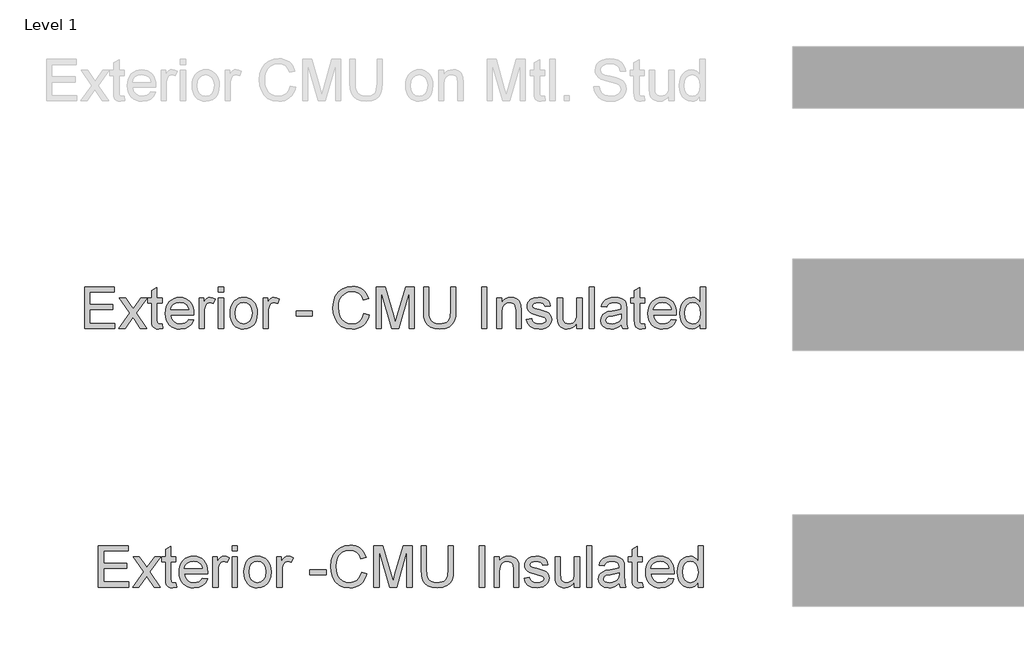
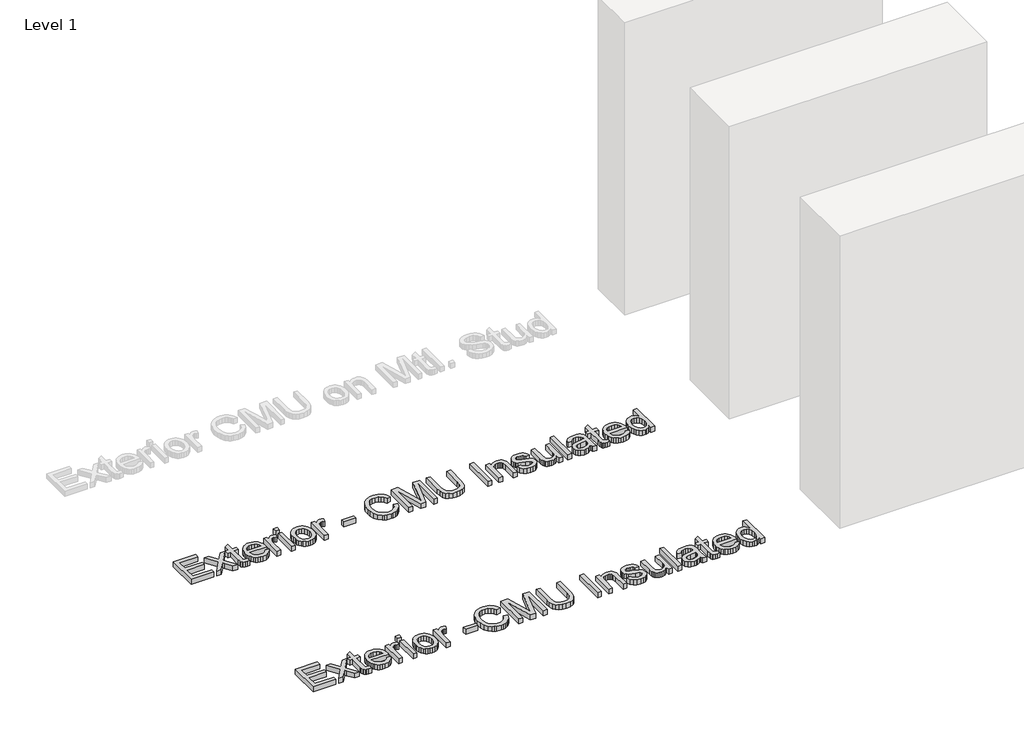
# One storey, part 20 of 42: 2 proxies.
"""IFC4 building model written with IfcOpenShell, lengths in millimetres."""

from ifc_helpers import new_model, si_unit, origin, origin_with_axes, place, context, project, spatial, polyline, outline, extrude, element, save

model = new_model("IFC4")

# Units and contexts
model_context = context("Model", 3, world=origin())
ifc_project = project(units=[si_unit("LENGTHUNIT", "METRE", prefix="MILLI")], contexts=[model_context])

# Site, building, storey
site = spatial("IfcSite", under=ifc_project)
building = spatial("IfcBuilding", under=site)
storey = spatial("IfcBuildingStorey", under=building, Name="Level 1", Elevation=0.0)

# Proxies
placement = place(None, origin())
element("IfcBuildingElementProxy", 1, Name="8\" Arial", ObjectType="8\" Arial", at=placement, inside=storey, context=model_context, shape_type="SweptSolid", body=[
    extrude(outline(polyline([(-4541.4204777, 3002.5650607), (-4541.4204777, 3307.1321548), (-4322.5128788, 3307.1321548), (-4322.5128788, 3269.061268), (-4503.3495909, 3269.061268), (-4503.3495909, 3178.642912), (-4332.0306005, 3178.642912), (-4332.0306005, 3140.5720252), (-4503.3495909, 3140.5720252), (-4503.3495909, 3040.6359475), (-4317.754018, 3040.6359475), (-4317.754018, 3002.5650607), (-4541.4204777, 3002.5650607)])), origin_with_axes(), (0.0, 0.0, 1.0), 50.8),
    extrude(outline(polyline([(-4289.2008529, 3002.5650607), (-4207.8540754, 3114.9931482), (-4284.4419921, 3226.2315204), (-4238.6379564, 3226.2315204), (-4201.6824277, 3172.6943359), (-4184.4315571, 3147.4128877), (-4169.4857598, 3168.0841895), (-4127.3995842, 3226.2315204), (-4081.5955486, 3226.2315204), (-4162.0500397, 3114.9931482), (-4084.5698366, 3002.5650607), (-4130.3738722, 3002.5650607), (-4176.9958371, 3070.1557562), (-4185.5469151, 3082.4990515), (-4243.3968173, 3002.5650607), (-4289.2008529, 3002.5650607)])), origin_with_axes(), (0.0, 0.0, 1.0), 50.8),
    extrude(outline(polyline([(-3970.3571763, 3034.3155854), (-3965.5983155, 3001.4497027), (-3994.0771233, 2997.8061999), (-4012.3504054, 2999.3862904), (-4025.9763624, 3004.126562), (-4035.6056199, 3011.4321569), (-4041.8888034, 3020.7082177), (-4045.3464132, 3036.639248), (-4046.4989498, 3063.9097513), (-4046.4989498, 3188.1606337), (-4075.0521149, 3188.1606337), (-4075.0521149, 3226.2315204), (-4046.4989498, 3226.2315204), (-4046.4989498, 3280.5866342), (-4008.4280631, 3302.9681516), (-4008.4280631, 3226.2315204), (-3970.3571763, 3226.2315204), (-3970.3571763, 3188.1606337), (-4008.4280631, 3188.1606337), (-4008.4280631, 3065.0251093), (-4006.4204187, 3045.3948083), (-3999.9141636, 3038.4424101), (-3986.9388321, 3035.8770867), (-3970.3571763, 3034.3155854)])), origin_with_axes(), (0.0, 0.0, 1.0), 50.8),
    extrude(outline(polyline([(-3775.6900249, 3069.1891126), (-3738.3627101, 3064.4302517), (-3751.8120688, 3036.3046406), (-3773.2734159, 3015.2801421), (-3802.2634295, 3002.1746854), (-3838.2987879, 2997.8061999), (-3861.9211411, 2999.6906902), (-3882.9688762, 3005.3441611), (-3901.4419932, 3014.7666126), (-3917.3404922, 3027.9580448), (-3930.1252834, 3044.5513188), (-3939.2572771, 3064.1792962), (-3944.7364734, 3086.8419767), (-3946.5628721, 3112.5393606), (-3944.7178841, 3139.1081179), (-3939.1829199, 3162.5259887), (-3929.9579797, 3182.7929733), (-3917.0430634, 3199.9090714), (-3901.1863904, 3213.5071445), (-3883.1361799, 3223.2200538), (-3862.892432, 3229.0477994), (-3840.4551467, 3230.9903813), (-3818.7405204, 3229.0524467), (-3799.1032485, 3223.2386431), (-3781.5433308, 3213.5489704), (-3766.0607674, 3199.9834286), (-3753.4223669, 3182.9045091), (-3744.394938, 3162.6747031), (-3738.9784807, 3139.2940109), (-3737.1729949, 3112.7624322), (-3737.3960665, 3102.5011385), (-3908.4919853, 3102.5011385), (-3901.9020784, 3074.0037413), (-3886.5937897, 3053.0536), (-3864.5004065, 3040.171215), (-3837.5552159, 3035.8770867), (-3817.2928787, 3037.8661418), (-3800.2279011, 3043.8333071), (-3786.3602832, 3054.1503687), (-3775.6900249, 3069.1891126)]), holes=[polyline([(-3908.4919853, 3140.5720252), (-3775.2438817, 3140.5720252), (-3780.3931178, 3160.685648), (-3790.4871078, 3175.0737664), (-3812.6827322, 3188.4580625), (-3840.6038611, 3192.9194945), (-3866.26639, 3189.3596435), (-3887.4860761, 3178.6800906), (-3902.2366858, 3162.0333723), (-3908.4919853, 3140.5720252)])]), origin_with_axes(), (0.0, 0.0, 1.0), 50.8),
    extrude(outline(polyline([(-3699.1021082, 3002.5650607), (-3699.1021082, 3226.2315204), (-3665.7900823, 3226.2315204), (-3665.7900823, 3193.1425661), (-3653.4839655, 3212.3267239), (-3642.1444924, 3223.6290184), (-3630.7678407, 3229.1500406), (-3618.3501882, 3230.9903813), (-3599.389102, 3228.0532719), (-3580.130587, 3219.2419436), (-3592.8456684, 3185.1119885), (-3606.2299645, 3190.967618), (-3619.6142606, 3192.9194945), (-3630.9816177, 3191.0419752), (-3641.1406702, 3185.4094173), (-3649.3478462, 3176.4493746), (-3654.8595737, 3164.5894011), (-3659.4883095, 3143.3232417), (-3661.0312214, 3120.123795), (-3661.0312214, 3002.5650607), (-3699.1021082, 3002.5650607)])), origin_with_axes(), (0.0, 0.0, 1.0), 50.8),
    extrude(outline(polyline([(-3556.3362828, 3269.061268), (-3556.3362828, 3307.1321548), (-3518.2653961, 3307.1321548), (-3518.2653961, 3269.061268), (-3556.3362828, 3269.061268)])), origin_with_axes(), (0.0, 0.0, 1.0), 50.8),
    extrude(outline(polyline([(-3556.3362828, 3002.5650607), (-3556.3362828, 3226.2315204), (-3518.2653961, 3226.2315204), (-3518.2653961, 3002.5650607), (-3556.3362828, 3002.5650607)])), origin_with_axes(), (0.0, 0.0, 1.0), 50.8),
    extrude(outline(polyline([(-3470.6767876, 3114.3982906), (-3468.6180226, 3143.3650676), (-3462.4417276, 3168.3258504), (-3452.1479027, 3189.280639), (-3437.7365477, 3206.2294335), (-3423.2275989, 3217.0623481), (-3407.2129168, 3224.8001443), (-3389.6925014, 3229.4428221), (-3370.6663527, 3230.9903813), (-3349.6627671, 3229.105891), (-3330.6714733, 3223.4524201), (-3313.6924713, 3214.0299685), (-3298.725761, 3200.8385364), (-3286.5102671, 3184.3242669), (-3277.7849143, 3164.9333031), (-3272.5497027, 3142.6656452), (-3270.8046321, 3117.521293), (-3273.890456, 3079.060031), (-3283.1479274, 3049.7818832), (-3298.3075017, 3027.8558036), (-3319.099634, 3011.4507462), (-3343.7955193, 3001.2173365), (-3370.6663527, 2997.8061999), (-3391.9766617, 2999.6837192), (-3411.1445538, 3005.3162772), (-3428.1700291, 3014.7038738), (-3443.0530876, 3027.846509), (-3455.1384563, 3044.5211112), (-3463.7708626, 3064.5046089), (-3468.9503064, 3087.797002), (-3470.6767876, 3114.3982906)]), holes=[polyline([(-3432.6059009, 3114.4726478), (-3428.2002367, 3080.0173799), (-3414.9832443, 3055.470209), (-3395.0926931, 3040.7753672), (-3370.6663527, 3035.8770867), (-3346.351548, 3040.8032512), (-3326.4981755, 3055.5817448), (-3313.281183, 3080.4542285), (-3308.8755189, 3115.662363), (-3313.309067, 3149.1138087), (-3326.6097113, 3173.3263721), (-3346.4909678, 3188.0212139), (-3370.6663527, 3192.9194945), (-3395.0926931, 3188.0398032), (-3414.9832443, 3173.4007293), (-3428.2002367, 3148.9093264), (-3432.6059009, 3114.4726478)])]), origin_with_axes(), (0.0, 0.0, 1.0), 50.8),
    extrude(outline(polyline([(-3227.9748845, 3002.5650607), (-3227.9748845, 3226.2315204), (-3194.6628586, 3226.2315204), (-3194.6628586, 3193.1425661), (-3182.3567419, 3212.3267239), (-3171.0172688, 3223.6290184), (-3159.6406171, 3229.1500406), (-3147.2229646, 3230.9903813), (-3128.2618784, 3228.0532719), (-3109.0033634, 3219.2419436), (-3121.7184447, 3185.1119885), (-3135.1027409, 3190.967618), (-3148.487037, 3192.9194945), (-3159.854394, 3191.0419752), (-3170.0134466, 3185.4094173), (-3178.2206226, 3176.4493746), (-3183.7323501, 3164.5894011), (-3188.3610859, 3143.3232417), (-3189.9039978, 3120.123795), (-3189.9039978, 3002.5650607), (-3227.9748845, 3002.5650607)])), origin_with_axes(), (0.0, 0.0, 1.0), 50.8),
    extrude(outline(polyline([(-2985.2729814, 3092.9834168), (-2985.2729814, 3131.0543035), (-2866.3014603, 3131.0543035), (-2866.3014603, 3092.9834168), (-2985.2729814, 3092.9834168)])), origin_with_axes(), (0.0, 0.0, 1.0), 50.8),
    extrude(outline(polyline([(-2485.5925927, 3110.829145), (-2447.521706, 3101.0139945), (-2455.0550199, 3077.338197), (-2465.0885946, 3056.6506296), (-2477.6224303, 3038.9512922), (-2492.6565268, 3024.2401847), (-2509.8516295, 3012.6753164), (-2528.8684835, 3004.4146961), (-2549.707089, 2999.4583239), (-2572.367446, 2997.8061999), (-2616.5263285, 3002.8067216), (-2635.1969569, 3009.0573738), (-2651.5950433, 3017.8082869), (-2678.4751714, 3042.2903952), (-2698.0682937, 3075.7325462), (-2710.0305084, 3115.0489161), (-2714.0179133, 3157.153681), (-2709.510008, 3201.5635191), (-2695.9862921, 3239.9132454), (-2674.1531591, 3270.9852606), (-2644.7170022, 3293.5619657), (-2609.8062965, 3307.3087532), (-2571.5495167, 3311.8910157), (-2549.7744753, 3310.408519), (-2529.8072432, 3305.9610289), (-2511.6478206, 3298.5485455), (-2495.2962074, 3288.1710686), (-2481.0219486, 3275.1027906), (-2469.0945888, 3259.6179036), (-2452.2805668, 3221.3983024), (-2490.3514536, 3212.3267239), (-2503.5498567, 3240.0898437), (-2521.5814779, 3259.1345818), (-2544.6693887, 3270.1487421), (-2573.0366608, 3273.8201289), (-2605.7352398, 3269.7490722), (-2632.5967785, 3257.5359019), (-2652.9799462, 3238.46328), (-2666.2434118, 3213.8138679), (-2673.5211229, 3185.948507), (-2675.9470265, 3157.2280382), (-2673.0749797, 3122.0570823), (-2664.458839, 3091.6449872), (-2649.7732919, 3067.1535842), (-2628.6930255, 3049.7447046), (-2603.4208719, 3039.3439911), (-2576.1596632, 3035.8770867), (-2544.3812545, 3040.5987689), (-2517.9007964, 3054.7638156), (-2497.9080041, 3078.2235125), (-2485.5925927, 3110.829145)])), origin_with_axes(), (0.0, 0.0, 1.0), 50.8),
    extrude(outline(polyline([(-2395.1742367, 3002.5650607), (-2395.1742367, 3307.1321548), (-2329.6655429, 3307.1321548), (-2267.3542087, 3092.4629164), (-2254.7878418, 3047.6255244), (-2241.180474, 3096.1807764), (-2179.9101407, 3307.1321548), (-2114.4014468, 3307.1321548), (-2114.4014468, 3002.5650607), (-2152.4723336, 3002.5650607), (-2152.4723336, 3269.061268), (-2228.9858931, 3002.5650607), (-2280.5897904, 3002.5650607), (-2357.1033499, 3269.061268), (-2357.1033499, 3002.5650607), (-2395.1742367, 3002.5650607)])), origin_with_axes(), (0.0, 0.0, 1.0), 50.8),
    extrude(outline(polyline([(-1847.9052395, 3307.1321548), (-1809.8343528, 3307.1321548), (-1809.8343528, 3131.4260896), (-1812.4182655, 3090.2786736), (-1820.1700037, 3058.5932115), (-1834.6510685, 3034.1482817), (-1857.4229612, 3014.7224631), (-1888.5414497, 3002.0352657), (-1928.0623019, 2997.8061999), (-1966.7187516, 3001.4868813), (-1997.6234631, 3012.5289256), (-2020.7857312, 3030.5512522), (-2036.2148503, 3055.1727802), (-2044.8867588, 3088.196672), (-2047.777395, 3131.4260896), (-2047.777395, 3307.1321548), (-2009.7065083, 3307.1321548), (-2009.7065083, 3132.7645192), (-2007.8289889, 3098.5509122), (-2002.196431, 3074.728724), (-1991.9909052, 3058.2307201), (-1976.3944823, 3045.9896659), (-1956.0577879, 3038.4052315), (-1931.6314475, 3035.8770867), (-1892.9099353, 3040.8776084), (-1878.4149284, 3047.1282606), (-1867.1637545, 3055.8791736), (-1858.7381542, 3068.1852904), (-1852.7198683, 3085.1015535), (-1847.9052395, 3132.7645192), (-1847.9052395, 3307.1321548)])), origin_with_axes(), (0.0, 0.0, 1.0), 50.8),
    extrude(outline(polyline([(-1619.479919, 3002.5650607), (-1619.479919, 3307.1321548), (-1581.4090322, 3307.1321548), (-1581.4090322, 3002.5650607), (-1619.479919, 3002.5650607)])), origin_with_axes(), (0.0, 0.0, 1.0), 50.8),
    extrude(outline(polyline([(-1510.0261195, 3002.5650607), (-1510.0261195, 3226.2315204), (-1471.9552328, 3226.2315204), (-1471.9552328, 3195.0014962), (-1458.7289457, 3210.7466334), (-1442.8443887, 3221.99316), (-1424.3015618, 3228.741076), (-1403.1004649, 3230.9903813), (-1384.3345664, 3229.1779245), (-1367.1487584, 3223.7405542), (-1352.816408, 3215.3567798), (-1342.6108822, 3204.7051108), (-1331.1970519, 3176.7096248), (-1329.1894074, 3139.9028104), (-1329.1894074, 3002.5650607), (-1367.2602942, 3002.5650607), (-1367.2602942, 3134.7721636), (-1371.647369, 3168.4559755), (-1377.7167756, 3178.4849029), (-1387.1508454, 3186.2645251), (-1399.2431852, 3191.2557522), (-1413.2874014, 3192.9194945), (-1435.585267, 3189.1830452), (-1454.5928264, 3177.9736972), (-1462.1888792, 3168.8231142), (-1467.6146312, 3156.3171625), (-1471.9552328, 3121.2391531), (-1471.9552328, 3002.5650607), (-1510.0261195, 3002.5650607)])), origin_with_axes(), (0.0, 0.0, 1.0), 50.8),
    extrude(outline(polyline([(-1291.1185207, 3069.1891126), (-1253.0476339, 3073.9479734), (-1247.04329, 3057.6637465), (-1235.4249774, 3045.6922371), (-1218.1183389, 3038.3308743), (-1195.0490174, 3035.8770867), (-1172.2585354, 3038.126392), (-1156.2345586, 3044.8743079), (-1146.7540155, 3054.6522798), (-1143.5938345, 3065.9917529), (-1146.7726048, 3075.6953676), (-1156.3089158, 3083.0939091), (-1195.4951606, 3093.9500604), (-1252.8245623, 3112.5765392), (-1267.3335111, 3121.9362518), (-1277.8457604, 3134.3260204), (-1284.231185, 3148.9557996), (-1286.3596598, 3165.0355443), (-1284.6494442, 3179.786154), (-1279.5187974, 3193.4028163), (-1271.4324518, 3205.3464417), (-1260.85514, 3215.0779403), (-1236.6518712, 3226.3430562), (-1203.8975243, 3230.9903813), (-1179.1179871, 3229.1221566), (-1157.5729882, 3223.5174826), (-1140.2477605, 3214.7247436), (-1128.1275368, 3203.292324), (-1120.0969591, 3188.3744106), (-1115.0406694, 3169.1251903), (-1153.1115562, 3164.3663295), (-1157.9168903, 3176.3471334), (-1167.4253173, 3185.3722387), (-1181.7297838, 3191.0326806), (-1200.9232362, 3192.9194945), (-1222.7842532, 3191.1163324), (-1237.3582646, 3185.7068461), (-1245.556146, 3177.89934), (-1248.2887731, 3168.9021187), (-1243.7529838, 3157.8228958), (-1229.5507585, 3149.4205321), (-1196.759233, 3141.3155972), (-1140.8797967, 3123.3955119), (-1126.1198923, 3114.8258445), (-1114.9291336, 3103.0959961), (-1107.8744942, 3088.168788), (-1105.5229477, 3070.0070418), (-1108.2834588, 3051.2318486), (-1116.564992, 3033.5720134), (-1130.0515293, 3018.4124391), (-1148.4270525, 3007.1380286), (-1170.622677, 3000.1391571), (-1195.5695178, 2997.8061999), (-1233.9564226, 3002.3048105), (-1261.970498, 3015.8006425), (-1280.671334, 3038.1449813), (-1291.1185207, 3069.1891126)])), origin_with_axes(), (0.0, 0.0, 1.0), 50.8),
    extrude(outline(polyline([(-919.9273748, 3002.5650607), (-919.9273748, 3041.0077335), (-933.7020462, 3022.1070625), (-949.7446123, 3008.6065833), (-968.0550729, 3000.5062957), (-988.6334282, 2997.8061999), (-1007.1762552, 2999.7023085), (-1024.4364204, 3005.3906344), (-1038.9174852, 3013.9417124), (-1049.123011, 3024.4260777), (-1055.9917574, 3037.1597484), (-1060.4624841, 3052.4587424), (-1062.6932001, 3087.8527699), (-1062.6932001, 3226.2315204), (-1024.6223134, 3226.2315204), (-1024.6223134, 3105.7728553), (-1022.3172402, 3066.9583965), (-1016.7683341, 3054.010949), (-1007.259907, 3044.1679145), (-994.4239952, 3037.9497936), (-978.8926349, 3035.8770867), (-962.4689882, 3037.9962669), (-947.1049316, 3044.3538075), (-934.4363236, 3054.3641457), (-926.0990224, 3067.4417184), (-921.4702867, 3085.3525091), (-919.9273748, 3109.8625013), (-919.9273748, 3226.2315204), (-881.856488, 3226.2315204), (-881.856488, 3002.5650607), (-919.9273748, 3002.5650607)])), origin_with_axes(), (0.0, 0.0, 1.0), 50.8),
    extrude(outline(polyline([(-829.5090187, 3002.5650607), (-829.5090187, 3307.1321548), (-791.438132, 3307.1321548), (-791.438132, 3002.5650607), (-829.5090187, 3002.5650607)])), origin_with_axes(), (0.0, 0.0, 1.0), 50.8),
    extrude(outline(polyline([(-591.5659765, 3031.1182258), (-609.7556067, 3015.521803), (-628.4843266, 3005.3162772), (-648.1796902, 2999.6837192), (-669.2692512, 2997.8061999), (-701.0848385, 3002.3233998), (-724.55383, 3015.8749997), (-739.0256001, 3036.453355), (-743.8495235, 3062.0508213), (-742.0277721, 3077.8331371), (-736.5625179, 3092.1654876), (-728.1322702, 3104.4344257), (-717.4155387, 3114.0265046), (-690.7584822, 3126.5185143), (-657.8182423, 3132.2440188), (-618.8922478, 3138.266952), (-591.7890481, 3145.3308861), (-591.5659765, 3153.807607), (-594.1870678, 3170.7982273), (-602.0503418, 3181.9146288), (-619.6358198, 3190.1682781), (-644.1365174, 3192.9194945), (-666.8154636, 3191.0884485), (-682.6535474, 3185.5953103), (-693.4539308, 3175.4362577), (-701.0197759, 3159.6074686), (-739.0906627, 3164.3663295), (-732.4821665, 3185.1863457), (-722.6205427, 3201.5449298), (-708.5856211, 3214.0555288), (-689.4572312, 3223.3315896), (-666.062597, 3229.0756834), (-639.2289421, 3230.9903813), (-613.4920561, 3229.298755), (-593.0902991, 3224.223876), (-577.7076532, 3216.5929683), (-567.0281003, 3207.2332557), (-559.9455769, 3195.6614163), (-555.3540198, 3181.3941284), (-553.4950897, 3148.0821025), (-553.4950897, 3100.7165657), (-551.5618025, 3034.5758356), (-543.9773681, 3002.5650607), (-582.0482548, 3002.5650607), (-588.1455453, 3015.8006425), (-591.5659765, 3031.1182258)]), holes=[polyline([(-591.5659765, 3107.2599993), (-652.9850243, 3095.5859188), (-685.7393712, 3089.4142712), (-700.5736327, 3079.3760491), (-705.7786368, 3064.7276805), (-702.9437685, 3053.4067967), (-694.4391637, 3044.1307359), (-680.4507153, 3037.940499), (-661.1643164, 3035.8770867), (-640.7160862, 3038.1542759), (-622.6472864, 3044.9858437), (-607.9989179, 3055.0519498), (-597.8119814, 3067.0327537), (-593.2947814, 3079.3760491), (-591.7890481, 3096.4782052), (-591.5659765, 3107.2599993)])]), origin_with_axes(), (0.0, 0.0, 1.0), 50.8),
    extrude(outline(polyline([(-420.2469861, 3034.3155854), (-415.4881252, 3001.4497027), (-443.9669331, 2997.8061999), (-462.2402152, 2999.3862904), (-475.8661722, 3004.126562), (-485.4954297, 3011.4321569), (-491.7786132, 3020.7082177), (-495.236223, 3036.639248), (-496.3887596, 3063.9097513), (-496.3887596, 3188.1606337), (-524.9419247, 3188.1606337), (-524.9419247, 3226.2315204), (-496.3887596, 3226.2315204), (-496.3887596, 3280.5866342), (-458.3178728, 3302.9681516), (-458.3178728, 3226.2315204), (-420.2469861, 3226.2315204), (-420.2469861, 3188.1606337), (-458.3178728, 3188.1606337), (-458.3178728, 3065.0251093), (-456.3102284, 3045.3948083), (-449.8039734, 3038.4424101), (-436.8286418, 3035.8770867), (-420.2469861, 3034.3155854)])), origin_with_axes(), (0.0, 0.0, 1.0), 50.8),
    extrude(outline(polyline([(-225.5798347, 3069.1891126), (-188.2525199, 3064.4302517), (-201.7018786, 3036.3046406), (-223.1632256, 3015.2801421), (-252.1532393, 3002.1746854), (-288.1885976, 2997.8061999), (-311.8109508, 2999.6906902), (-332.858686, 3005.3441611), (-351.331803, 3014.7666126), (-367.230302, 3027.9580448), (-380.0150932, 3044.5513188), (-389.1470869, 3064.1792962), (-394.6262831, 3086.8419767), (-396.4526819, 3112.5393606), (-394.6076938, 3139.1081179), (-389.0727297, 3162.5259887), (-379.8477895, 3182.7929733), (-366.9328732, 3199.9090714), (-351.0762001, 3213.5071445), (-333.0259897, 3223.2200538), (-312.7822418, 3229.0477994), (-290.3449565, 3230.9903813), (-268.6303302, 3229.0524467), (-248.9930582, 3223.2386431), (-231.4331405, 3213.5489704), (-215.9505772, 3199.9834286), (-203.3121767, 3182.9045091), (-194.2847478, 3162.6747031), (-188.8682905, 3139.2940109), (-187.0628047, 3112.7624322), (-187.2858763, 3102.5011385), (-358.3817951, 3102.5011385), (-351.7918882, 3074.0037413), (-336.4835995, 3053.0536), (-314.3902162, 3040.171215), (-287.4450256, 3035.8770867), (-267.1826884, 3037.8661418), (-250.1177109, 3043.8333071), (-236.250093, 3054.1503687), (-225.5798347, 3069.1891126)]), holes=[polyline([(-358.3817951, 3140.5720252), (-225.1336914, 3140.5720252), (-230.2829276, 3160.685648), (-240.3769176, 3175.0737664), (-262.572542, 3188.4580625), (-290.4936709, 3192.9194945), (-316.1561998, 3189.3596435), (-337.3758859, 3178.6800906), (-352.1264956, 3162.0333723), (-358.3817951, 3140.5720252)])]), origin_with_axes(), (0.0, 0.0, 1.0), 50.8),
    extrude(outline(polyline([(-10.9849534, 3002.5650607), (-10.9849534, 3038.4795887), (-22.3755471, 3020.6849811), (-36.1734552, 3007.9745471), (-52.3786776, 3000.3482867), (-70.9912144, 2997.8061999), (-95.6034478, 3001.4868813), (-118.1336796, 3012.5289256), (-137.2063016, 3030.1608768), (-151.4457056, 3053.611279), (-160.3128017, 3081.9320778), (-163.2685005, 3114.175219), (-160.545168, 3146.0186902), (-152.3751706, 3174.7763376), (-138.7678028, 3198.8123027), (-119.7323595, 3216.4907272), (-96.7095112, 3227.3654678), (-71.1399288, 3230.9903813), (-52.51345, 3228.3971739), (-36.0433301, 3220.6175518), (-22.0827656, 3208.6925157), (-10.9849534, 3193.6630665), (-10.9849534, 3307.1321548), (27.0859333, 3307.1321548), (27.0859333, 3002.5650607), (-10.9849534, 3002.5650607)]), holes=[polyline([(-125.1976137, 3114.3239334), (-120.9034854, 3079.8872548), (-108.0211003, 3055.3958518), (-89.3016751, 3040.7567779), (-67.496426, 3035.8770867), (-45.7004715, 3040.5337063), (-27.4550734, 3054.5035654), (-15.1024834, 3078.0469141), (-10.9849534, 3111.4240026), (-15.1768406, 3147.9147988), (-27.7525022, 3173.2148363), (-46.4626328, 3187.99333), (-69.0579272, 3192.9194945), (-91.0862479, 3188.1885176), (-109.1364584, 3173.995587), (-121.1823249, 3149.6157198), (-125.1976137, 3114.3239334)])]), origin_with_axes(), (0.0, 0.0, 1.0), 50.8),
])
element("IfcBuildingElementProxy", 2, Name="8\" Arial", ObjectType="8\" Arial", at=placement, inside=storey, context=model_context, shape_type="SweptSolid", body=[
    extrude(outline(polyline([(-4439.8204777, 1097.5650607), (-4439.8204777, 1402.1321548), (-4220.9128788, 1402.1321548), (-4220.9128788, 1364.061268), (-4401.7495909, 1364.061268), (-4401.7495909, 1273.642912), (-4230.4306005, 1273.642912), (-4230.4306005, 1235.5720252), (-4401.7495909, 1235.5720252), (-4401.7495909, 1135.6359475), (-4216.154018, 1135.6359475), (-4216.154018, 1097.5650607), (-4439.8204777, 1097.5650607)])), origin_with_axes(), (0.0, 0.0, 1.0), 50.8),
    extrude(outline(polyline([(-4187.6008529, 1097.5650607), (-4106.2540754, 1209.9931482), (-4182.8419921, 1321.2315204), (-4137.0379564, 1321.2315204), (-4100.0824277, 1267.6943359), (-4082.8315571, 1242.4128877), (-4067.8857598, 1263.0841895), (-4025.7995842, 1321.2315204), (-3979.9955486, 1321.2315204), (-4060.4500397, 1209.9931482), (-3982.9698366, 1097.5650607), (-4028.7738722, 1097.5650607), (-4075.3958371, 1165.1557562), (-4083.9469151, 1177.4990515), (-4141.7968173, 1097.5650607), (-4187.6008529, 1097.5650607)])), origin_with_axes(), (0.0, 0.0, 1.0), 50.8),
    extrude(outline(polyline([(-3868.7571763, 1129.3155854), (-3863.9983155, 1096.4497027), (-3892.4771233, 1092.8061999), (-3910.7504054, 1094.3862904), (-3924.3763624, 1099.126562), (-3934.0056199, 1106.4321569), (-3940.2888034, 1115.7082177), (-3943.7464132, 1131.639248), (-3944.8989498, 1158.9097513), (-3944.8989498, 1283.1606337), (-3973.4521149, 1283.1606337), (-3973.4521149, 1321.2315204), (-3944.8989498, 1321.2315204), (-3944.8989498, 1375.5866342), (-3906.8280631, 1397.9681516), (-3906.8280631, 1321.2315204), (-3868.7571763, 1321.2315204), (-3868.7571763, 1283.1606337), (-3906.8280631, 1283.1606337), (-3906.8280631, 1160.0251093), (-3904.8204187, 1140.3948083), (-3898.3141636, 1133.4424101), (-3885.3388321, 1130.8770867), (-3868.7571763, 1129.3155854)])), origin_with_axes(), (0.0, 0.0, 1.0), 50.8),
    extrude(outline(polyline([(-3674.0900249, 1164.1891126), (-3636.7627101, 1159.4302517), (-3650.2120688, 1131.3046406), (-3671.6734159, 1110.2801421), (-3700.6634295, 1097.1746854), (-3736.6987879, 1092.8061999), (-3760.3211411, 1094.6906902), (-3781.3688762, 1100.3441611), (-3799.8419932, 1109.7666126), (-3815.7404922, 1122.9580448), (-3828.5252834, 1139.5513188), (-3837.6572771, 1159.1792962), (-3843.1364734, 1181.8419767), (-3844.9628721, 1207.5393606), (-3843.1178841, 1234.1081179), (-3837.5829199, 1257.5259887), (-3828.3579797, 1277.7929733), (-3815.4430634, 1294.9090714), (-3799.5863904, 1308.5071445), (-3781.5361799, 1318.2200538), (-3761.292432, 1324.0477994), (-3738.8551467, 1325.9903813), (-3717.1405204, 1324.0524467), (-3697.5032485, 1318.2386431), (-3679.9433308, 1308.5489704), (-3664.4607674, 1294.9834286), (-3651.8223669, 1277.9045091), (-3642.794938, 1257.6747031), (-3637.3784807, 1234.2940109), (-3635.5729949, 1207.7624322), (-3635.7960665, 1197.5011385), (-3806.8919853, 1197.5011385), (-3800.3020784, 1169.0037413), (-3784.9937897, 1148.0536), (-3762.9004065, 1135.171215), (-3735.9552159, 1130.8770867), (-3715.6928787, 1132.8661418), (-3698.6279011, 1138.8333071), (-3684.7602832, 1149.1503687), (-3674.0900249, 1164.1891126)]), holes=[polyline([(-3806.8919853, 1235.5720252), (-3673.6438817, 1235.5720252), (-3678.7931178, 1255.685648), (-3688.8871078, 1270.0737664), (-3711.0827322, 1283.4580625), (-3739.0038611, 1287.9194945), (-3764.66639, 1284.3596435), (-3785.8860761, 1273.6800906), (-3800.6366858, 1257.0333723), (-3806.8919853, 1235.5720252)])]), origin_with_axes(), (0.0, 0.0, 1.0), 50.8),
    extrude(outline(polyline([(-3597.5021082, 1097.5650607), (-3597.5021082, 1321.2315204), (-3564.1900823, 1321.2315204), (-3564.1900823, 1288.1425661), (-3551.8839655, 1307.3267239), (-3540.5444924, 1318.6290184), (-3529.1678407, 1324.1500406), (-3516.7501882, 1325.9903813), (-3497.789102, 1323.0532719), (-3478.530587, 1314.2419436), (-3491.2456684, 1280.1119885), (-3504.6299645, 1285.967618), (-3518.0142606, 1287.9194945), (-3529.3816177, 1286.0419752), (-3539.5406702, 1280.4094173), (-3547.7478462, 1271.4493746), (-3553.2595737, 1259.5894011), (-3557.8883095, 1238.3232417), (-3559.4312214, 1215.123795), (-3559.4312214, 1097.5650607), (-3597.5021082, 1097.5650607)])), origin_with_axes(), (0.0, 0.0, 1.0), 50.8),
    extrude(outline(polyline([(-3454.7362828, 1364.061268), (-3454.7362828, 1402.1321548), (-3416.6653961, 1402.1321548), (-3416.6653961, 1364.061268), (-3454.7362828, 1364.061268)])), origin_with_axes(), (0.0, 0.0, 1.0), 50.8),
    extrude(outline(polyline([(-3454.7362828, 1097.5650607), (-3454.7362828, 1321.2315204), (-3416.6653961, 1321.2315204), (-3416.6653961, 1097.5650607), (-3454.7362828, 1097.5650607)])), origin_with_axes(), (0.0, 0.0, 1.0), 50.8),
    extrude(outline(polyline([(-3369.0767876, 1209.3982906), (-3367.0180226, 1238.3650676), (-3360.8417276, 1263.3258504), (-3350.5479027, 1284.280639), (-3336.1365477, 1301.2294335), (-3321.6275989, 1312.0623481), (-3305.6129168, 1319.8001443), (-3288.0925014, 1324.4428221), (-3269.0663527, 1325.9903813), (-3248.0627671, 1324.105891), (-3229.0714733, 1318.4524201), (-3212.0924713, 1309.0299685), (-3197.125761, 1295.8385364), (-3184.9102671, 1279.3242669), (-3176.1849143, 1259.9333031), (-3170.9497027, 1237.6656452), (-3169.2046321, 1212.521293), (-3172.290456, 1174.060031), (-3181.5479274, 1144.7818832), (-3196.7075017, 1122.8558036), (-3217.499634, 1106.4507462), (-3242.1955193, 1096.2173365), (-3269.0663527, 1092.8061999), (-3290.3766617, 1094.6837192), (-3309.5445538, 1100.3162772), (-3326.5700291, 1109.7038738), (-3341.4530876, 1122.846509), (-3353.5384563, 1139.5211112), (-3362.1708626, 1159.5046089), (-3367.3503064, 1182.797002), (-3369.0767876, 1209.3982906)]), holes=[polyline([(-3331.0059009, 1209.4726478), (-3326.6002367, 1175.0173799), (-3313.3832443, 1150.470209), (-3293.4926931, 1135.7753672), (-3269.0663527, 1130.8770867), (-3244.751548, 1135.8032512), (-3224.8981755, 1150.5817448), (-3211.681183, 1175.4542285), (-3207.2755189, 1210.662363), (-3211.709067, 1244.1138087), (-3225.0097113, 1268.3263721), (-3244.8909678, 1283.0212139), (-3269.0663527, 1287.9194945), (-3293.4926931, 1283.0398032), (-3313.3832443, 1268.4007293), (-3326.6002367, 1243.9093264), (-3331.0059009, 1209.4726478)])]), origin_with_axes(), (0.0, 0.0, 1.0), 50.8),
    extrude(outline(polyline([(-3126.3748845, 1097.5650607), (-3126.3748845, 1321.2315204), (-3093.0628586, 1321.2315204), (-3093.0628586, 1288.1425661), (-3080.7567419, 1307.3267239), (-3069.4172688, 1318.6290184), (-3058.0406171, 1324.1500406), (-3045.6229646, 1325.9903813), (-3026.6618784, 1323.0532719), (-3007.4033634, 1314.2419436), (-3020.1184447, 1280.1119885), (-3033.5027409, 1285.967618), (-3046.887037, 1287.9194945), (-3058.254394, 1286.0419752), (-3068.4134466, 1280.4094173), (-3076.6206226, 1271.4493746), (-3082.1323501, 1259.5894011), (-3086.7610859, 1238.3232417), (-3088.3039978, 1215.123795), (-3088.3039978, 1097.5650607), (-3126.3748845, 1097.5650607)])), origin_with_axes(), (0.0, 0.0, 1.0), 50.8),
    extrude(outline(polyline([(-2883.6729814, 1187.9834168), (-2883.6729814, 1226.0543035), (-2764.7014603, 1226.0543035), (-2764.7014603, 1187.9834168), (-2883.6729814, 1187.9834168)])), origin_with_axes(), (0.0, 0.0, 1.0), 50.8),
    extrude(outline(polyline([(-2502.9641139, 1205.829145), (-2464.8932271, 1196.0139945), (-2472.426541, 1172.338197), (-2482.4601158, 1151.6506296), (-2494.9939514, 1133.9512922), (-2510.0280479, 1119.2401847), (-2527.2231506, 1107.6753164), (-2546.2400047, 1099.4146961), (-2567.0786102, 1094.4583239), (-2589.7389671, 1092.8061999), (-2633.8978496, 1097.8067216), (-2652.568478, 1104.0573738), (-2668.9665644, 1112.8082869), (-2695.8466925, 1137.2903952), (-2715.4398149, 1170.7325462), (-2727.4020295, 1210.0489161), (-2731.3894344, 1252.153681), (-2726.8815291, 1296.5635191), (-2713.3578132, 1334.9132454), (-2691.5246802, 1365.9852606), (-2662.0885234, 1388.5619657), (-2627.1778176, 1402.3087532), (-2588.9210379, 1406.8910157), (-2567.1459964, 1405.408519), (-2547.1787643, 1400.9610289), (-2529.0193417, 1393.5485455), (-2512.6677285, 1383.1710686), (-2498.3934697, 1370.1027906), (-2486.46611, 1354.6179036), (-2469.6520879, 1316.3983024), (-2507.7229747, 1307.3267239), (-2520.9213778, 1335.0898437), (-2538.952999, 1354.1345818), (-2562.0409098, 1365.1487421), (-2590.4081819, 1368.8201289), (-2623.1067609, 1364.7490722), (-2649.9682996, 1352.5359019), (-2670.3514673, 1333.46328), (-2683.614933, 1308.8138679), (-2690.892644, 1280.948507), (-2693.3185476, 1252.2280382), (-2690.4465008, 1217.0570823), (-2681.8303601, 1186.6449872), (-2667.144813, 1162.1535842), (-2646.0645466, 1144.7447046), (-2620.792393, 1134.3439911), (-2593.5311843, 1130.8770867), (-2561.7527757, 1135.5987689), (-2535.2723176, 1149.7638156), (-2515.2795252, 1173.2235125), (-2502.9641139, 1205.829145)])), origin_with_axes(), (0.0, 0.0, 1.0), 50.8),
    extrude(outline(polyline([(-2412.5457578, 1097.5650607), (-2412.5457578, 1402.1321548), (-2347.037064, 1402.1321548), (-2284.7257298, 1187.4629164), (-2272.1593629, 1142.6255244), (-2258.5519952, 1191.1807764), (-2197.2816618, 1402.1321548), (-2131.772968, 1402.1321548), (-2131.772968, 1097.5650607), (-2169.8438547, 1097.5650607), (-2169.8438547, 1364.061268), (-2246.3574142, 1097.5650607), (-2297.9613115, 1097.5650607), (-2374.474871, 1364.061268), (-2374.474871, 1097.5650607), (-2412.5457578, 1097.5650607)])), origin_with_axes(), (0.0, 0.0, 1.0), 50.8),
    extrude(outline(polyline([(-1865.2767607, 1402.1321548), (-1827.2058739, 1402.1321548), (-1827.2058739, 1226.4260896), (-1829.7897866, 1185.2786736), (-1837.5415248, 1153.5932115), (-1852.0225896, 1129.1482817), (-1874.7944823, 1109.7224631), (-1905.9129708, 1097.0352657), (-1945.433823, 1092.8061999), (-1984.0902727, 1096.4868813), (-2014.9949843, 1107.5289256), (-2038.1572523, 1125.5512522), (-2053.5863714, 1150.1727802), (-2062.25828, 1183.196672), (-2065.1489161, 1226.4260896), (-2065.1489161, 1402.1321548), (-2027.0780294, 1402.1321548), (-2027.0780294, 1227.7645192), (-2025.2005101, 1193.5509122), (-2019.5679521, 1169.728724), (-2009.3624263, 1153.2307201), (-1993.7660035, 1140.9896659), (-1973.4293091, 1133.4052315), (-1949.0029686, 1130.8770867), (-1910.2814564, 1135.8776084), (-1895.7864496, 1142.1282606), (-1884.5352756, 1150.8791736), (-1876.1096753, 1163.1852904), (-1870.0913894, 1180.1015535), (-1865.2767607, 1227.7645192), (-1865.2767607, 1402.1321548)])), origin_with_axes(), (0.0, 0.0, 1.0), 50.8),
    extrude(outline(polyline([(-1636.8514401, 1097.5650607), (-1636.8514401, 1402.1321548), (-1598.7805533, 1402.1321548), (-1598.7805533, 1097.5650607), (-1636.8514401, 1097.5650607)])), origin_with_axes(), (0.0, 0.0, 1.0), 50.8),
    extrude(outline(polyline([(-1527.3976407, 1097.5650607), (-1527.3976407, 1321.2315204), (-1489.3267539, 1321.2315204), (-1489.3267539, 1290.0014962), (-1476.1004668, 1305.7466334), (-1460.2159098, 1316.99316), (-1441.6730829, 1323.741076), (-1420.4719861, 1325.9903813), (-1401.7060875, 1324.1779245), (-1384.5202795, 1318.7405542), (-1370.1879291, 1310.3567798), (-1359.9824033, 1299.7051108), (-1348.568573, 1271.7096248), (-1346.5609286, 1234.9028104), (-1346.5609286, 1097.5650607), (-1384.6318153, 1097.5650607), (-1384.6318153, 1229.7721636), (-1389.0188902, 1263.4559755), (-1395.0882967, 1273.4849029), (-1404.5223665, 1281.2645251), (-1416.6147063, 1286.2557522), (-1430.6589226, 1287.9194945), (-1452.9567881, 1284.1830452), (-1471.9643475, 1272.9736972), (-1479.5604003, 1263.8231142), (-1484.9861523, 1251.3171625), (-1489.3267539, 1216.2391531), (-1489.3267539, 1097.5650607), (-1527.3976407, 1097.5650607)])), origin_with_axes(), (0.0, 0.0, 1.0), 50.8),
    extrude(outline(polyline([(-1308.4900418, 1164.1891126), (-1270.419155, 1168.9479734), (-1264.4148111, 1152.6637465), (-1252.7964985, 1140.6922371), (-1235.48986, 1133.3308743), (-1212.4205385, 1130.8770867), (-1189.6300565, 1133.126392), (-1173.6060797, 1139.8743079), (-1164.1255366, 1149.6522798), (-1160.9653556, 1160.9917529), (-1164.1441259, 1170.6953676), (-1173.6804369, 1178.0939091), (-1212.8666817, 1188.9500604), (-1270.1960834, 1207.5765392), (-1284.7050322, 1216.9362518), (-1295.2172815, 1229.3260204), (-1301.6027061, 1243.9557996), (-1303.731181, 1260.0355443), (-1302.0209653, 1274.786154), (-1296.8903185, 1288.4028163), (-1288.8039729, 1300.3464417), (-1278.2266611, 1310.0779403), (-1254.0233923, 1321.3430562), (-1221.2690454, 1325.9903813), (-1196.4895083, 1324.1221566), (-1174.9445094, 1318.5174826), (-1157.6192816, 1309.7247436), (-1145.4990579, 1298.292324), (-1137.4684802, 1283.3744106), (-1132.4121905, 1264.1251903), (-1170.4830773, 1259.3663295), (-1175.2884114, 1271.3471334), (-1184.7968384, 1280.3722387), (-1199.1013049, 1286.0326806), (-1218.2947574, 1287.9194945), (-1240.1557744, 1286.1163324), (-1254.7297857, 1280.7068461), (-1262.9276671, 1272.89934), (-1265.6602942, 1263.9021187), (-1261.124505, 1252.8228958), (-1246.9222796, 1244.4205321), (-1214.1307541, 1236.3155972), (-1158.2513178, 1218.3955119), (-1143.4914135, 1209.8258445), (-1132.3006547, 1198.0959961), (-1125.2460153, 1183.168788), (-1122.8944689, 1165.0070418), (-1125.6549799, 1146.2318486), (-1133.9365132, 1128.5720134), (-1147.4230504, 1113.4124391), (-1165.7985737, 1102.1380286), (-1187.9941981, 1095.1391571), (-1212.9410389, 1092.8061999), (-1251.3279438, 1097.3048105), (-1279.3420191, 1110.8006425), (-1298.0428551, 1133.1449813), (-1308.4900418, 1164.1891126)])), origin_with_axes(), (0.0, 0.0, 1.0), 50.8),
    extrude(outline(polyline([(-937.2988959, 1097.5650607), (-937.2988959, 1136.0077335), (-951.0735673, 1117.1070625), (-967.1161334, 1103.6065833), (-985.4265941, 1095.5062957), (-1006.0049494, 1092.8061999), (-1024.5477763, 1094.7023085), (-1041.8079415, 1100.3906344), (-1056.2890063, 1108.9417124), (-1066.4945321, 1119.4260777), (-1073.3632785, 1132.1597484), (-1077.8340052, 1147.4587424), (-1080.0647213, 1182.8527699), (-1080.0647213, 1321.2315204), (-1041.9938345, 1321.2315204), (-1041.9938345, 1200.7728553), (-1039.6887613, 1161.9583965), (-1034.1398552, 1149.010949), (-1024.6314281, 1139.1679145), (-1011.7955164, 1132.9497936), (-996.2641561, 1130.8770867), (-979.8405094, 1132.9962669), (-964.4764528, 1139.3538075), (-951.8078447, 1149.3641457), (-943.4705436, 1162.4417184), (-938.8418078, 1180.3525091), (-937.2988959, 1204.8625013), (-937.2988959, 1321.2315204), (-899.2280092, 1321.2315204), (-899.2280092, 1097.5650607), (-937.2988959, 1097.5650607)])), origin_with_axes(), (0.0, 0.0, 1.0), 50.8),
    extrude(outline(polyline([(-846.8805399, 1097.5650607), (-846.8805399, 1402.1321548), (-808.8096531, 1402.1321548), (-808.8096531, 1097.5650607), (-846.8805399, 1097.5650607)])), origin_with_axes(), (0.0, 0.0, 1.0), 50.8),
    extrude(outline(polyline([(-608.9374976, 1126.1182258), (-627.1271278, 1110.521803), (-645.8558478, 1100.3162772), (-665.5512113, 1094.6837192), (-686.6407724, 1092.8061999), (-718.4563596, 1097.3233998), (-741.9253511, 1110.8749997), (-756.3971213, 1131.453355), (-761.2210447, 1157.0508213), (-759.3992932, 1172.8331371), (-753.934039, 1187.1654876), (-745.5037914, 1199.4344257), (-734.7870598, 1209.0265046), (-708.1300034, 1221.5185143), (-675.1897634, 1227.2440188), (-636.2637689, 1233.266952), (-609.1605692, 1240.3308861), (-608.9374976, 1248.807607), (-611.5585889, 1265.7982273), (-619.4218629, 1276.9146288), (-637.0073409, 1285.1682781), (-661.5080385, 1287.9194945), (-684.1869847, 1286.0884485), (-700.0250685, 1280.5953103), (-710.8254519, 1270.4362577), (-718.3912971, 1254.6074686), (-756.4621838, 1259.3663295), (-749.8536876, 1280.1863457), (-739.9920639, 1296.5449298), (-725.9571422, 1309.0555288), (-706.8287523, 1318.3315896), (-683.4341181, 1324.0756834), (-656.6004633, 1325.9903813), (-630.8635772, 1324.298755), (-610.4618202, 1319.223876), (-595.0791743, 1311.5929683), (-584.3996214, 1302.2332557), (-577.317098, 1290.6614163), (-572.7255409, 1276.3941284), (-570.8666109, 1243.0821025), (-570.8666109, 1195.7165657), (-568.9333236, 1129.5758356), (-561.3488892, 1097.5650607), (-599.4197759, 1097.5650607), (-605.5170664, 1110.8006425), (-608.9374976, 1126.1182258)]), holes=[polyline([(-608.9374976, 1202.2599993), (-670.3565454, 1190.5859188), (-703.1108923, 1184.4142712), (-717.9451538, 1174.3760491), (-723.1501579, 1159.7276805), (-720.3152896, 1148.4067967), (-711.8106848, 1139.1307359), (-697.8222364, 1132.940499), (-678.5358375, 1130.8770867), (-658.0876073, 1133.1542759), (-640.0188075, 1139.9858437), (-625.370439, 1150.0519498), (-615.1835025, 1162.0327537), (-610.6663025, 1174.3760491), (-609.1605692, 1191.4782052), (-608.9374976, 1202.2599993)])]), origin_with_axes(), (0.0, 0.0, 1.0), 50.8),
    extrude(outline(polyline([(-437.6185072, 1129.3155854), (-432.8596464, 1096.4497027), (-461.3384542, 1092.8061999), (-479.6117363, 1094.3862904), (-493.2376933, 1099.126562), (-502.8669508, 1106.4321569), (-509.1501343, 1115.7082177), (-512.6077441, 1131.639248), (-513.7602807, 1158.9097513), (-513.7602807, 1283.1606337), (-542.3134458, 1283.1606337), (-542.3134458, 1321.2315204), (-513.7602807, 1321.2315204), (-513.7602807, 1375.5866342), (-475.689394, 1397.9681516), (-475.689394, 1321.2315204), (-437.6185072, 1321.2315204), (-437.6185072, 1283.1606337), (-475.689394, 1283.1606337), (-475.689394, 1160.0251093), (-473.6817495, 1140.3948083), (-467.1754945, 1133.4424101), (-454.200163, 1130.8770867), (-437.6185072, 1129.3155854)])), origin_with_axes(), (0.0, 0.0, 1.0), 50.8),
    extrude(outline(polyline([(-242.9513558, 1164.1891126), (-205.624041, 1159.4302517), (-219.0733997, 1131.3046406), (-240.5347468, 1110.2801421), (-269.5247604, 1097.1746854), (-305.5601188, 1092.8061999), (-329.182472, 1094.6906902), (-350.2302071, 1100.3441611), (-368.7033241, 1109.7666126), (-384.6018231, 1122.9580448), (-397.3866143, 1139.5513188), (-406.518608, 1159.1792962), (-411.9978042, 1181.8419767), (-413.824203, 1207.5393606), (-411.9792149, 1234.1081179), (-406.4442508, 1257.5259887), (-397.2193106, 1277.7929733), (-384.3043943, 1294.9090714), (-368.4477213, 1308.5071445), (-350.3975108, 1318.2200538), (-330.1537629, 1324.0477994), (-307.7164776, 1325.9903813), (-286.0018513, 1324.0524467), (-266.3645793, 1318.2386431), (-248.8046617, 1308.5489704), (-233.3220983, 1294.9834286), (-220.6836978, 1277.9045091), (-211.6562689, 1257.6747031), (-206.2398116, 1234.2940109), (-204.4343258, 1207.7624322), (-204.6573974, 1197.5011385), (-375.7533162, 1197.5011385), (-369.1634093, 1169.0037413), (-353.8551206, 1148.0536), (-331.7617374, 1135.171215), (-304.8165468, 1130.8770867), (-284.5542096, 1132.8661418), (-267.489232, 1138.8333071), (-253.6216141, 1149.1503687), (-242.9513558, 1164.1891126)]), holes=[polyline([(-375.7533162, 1235.5720252), (-242.5052126, 1235.5720252), (-247.6544487, 1255.685648), (-257.7484387, 1270.0737664), (-279.9440631, 1283.4580625), (-307.865192, 1287.9194945), (-333.5277209, 1284.3596435), (-354.747407, 1273.6800906), (-369.4980167, 1257.0333723), (-375.7533162, 1235.5720252)])]), origin_with_axes(), (0.0, 0.0, 1.0), 50.8),
    extrude(outline(polyline([(-28.3564746, 1097.5650607), (-28.3564746, 1133.4795887), (-39.7470682, 1115.6849811), (-53.5449763, 1102.9745471), (-69.7501987, 1095.3482867), (-88.3627355, 1092.8061999), (-112.9749689, 1096.4868813), (-135.5052008, 1107.5289256), (-154.5778227, 1125.1608768), (-168.8172267, 1148.611279), (-177.6843229, 1176.9320778), (-180.6400216, 1209.175219), (-177.9166891, 1241.0186902), (-169.7466917, 1269.7763376), (-156.139324, 1293.8123027), (-137.1038806, 1311.4907272), (-114.0810323, 1322.3654678), (-88.5114499, 1325.9903813), (-69.8849711, 1323.3971739), (-53.4148512, 1315.6175518), (-39.4542868, 1303.6925157), (-28.3564746, 1288.6630665), (-28.3564746, 1402.1321548), (9.7144122, 1402.1321548), (9.7144122, 1097.5650607), (-28.3564746, 1097.5650607)]), holes=[polyline([(-142.5691348, 1209.3239334), (-138.2750065, 1174.8872548), (-125.3926215, 1150.3958518), (-106.6731962, 1135.7567779), (-84.8679471, 1130.8770867), (-63.0719926, 1135.5337063), (-44.8265945, 1149.5035654), (-32.4740045, 1173.0469141), (-28.3564746, 1206.4240026), (-32.5483617, 1242.9147988), (-45.1240233, 1268.2148363), (-63.8341539, 1282.99333), (-86.4294483, 1287.9194945), (-108.457769, 1283.1885176), (-126.5079795, 1268.995587), (-138.553846, 1244.6157198), (-142.5691348, 1209.3239334)])]), origin_with_axes(), (0.0, 0.0, 1.0), 50.8),
])

save(model, "model.ifc")

# Revit data of these elements
# Elements 1, 2 (IfcBuildingElementProxy, "8\" Arial")
#   Phase Created = New Construction
